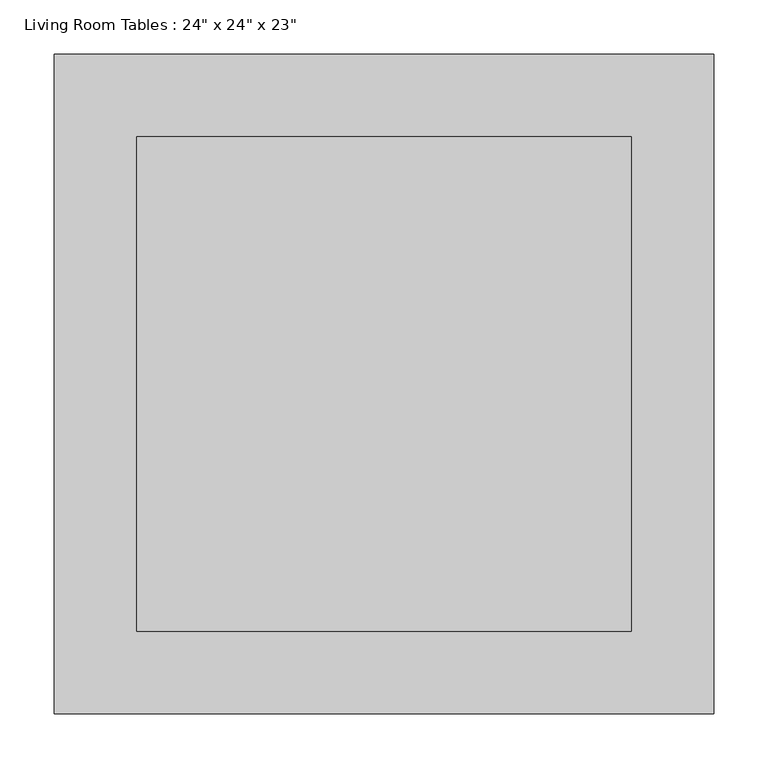
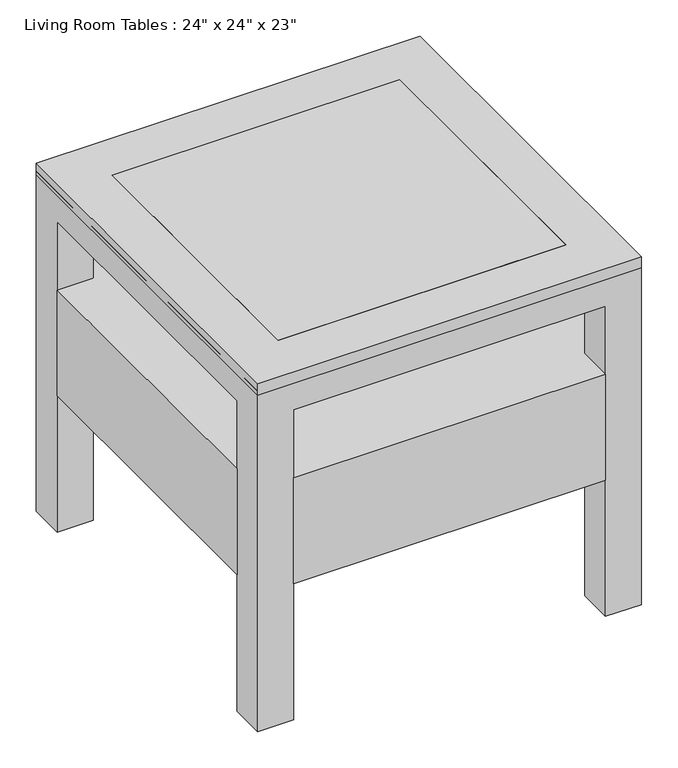
"""IFC4 building model written with IfcOpenShell, lengths in millimetres: furniture geometry."""

from ifc_helpers import new_model, si_unit, frame, origin, place, context, project, spatial, polyline, outline, extrude, faceted_brep, source, transform, mapped, element, save


def furniture_79813b58(model_context):
    return source(origin(), model_context, "Body", "SolidModel", [
        extrude(outline(polyline([(265.9157667, 400.0110778), (265.9157667, 342.8610778), (323.0657667, 342.8610778), (323.0657667, -152.4389222), (265.9157667, -152.4389222), (265.9157667, -209.5889222), (-229.3842333, -209.5889222), (-229.3842333, -152.4389222), (-286.5342333, -152.4389222), (-286.5342333, 342.8610778), (-229.3842333, 342.8610778), (-229.3842333, 400.0110778), (265.9157667, 400.0110778)])), frame((0.0, 0.0, 228.6), z_axis=(0.0, 0.0, 1.0), x_axis=(1.0, 0.0, 0.0)), (0.0, 0.0, 1.0), 177.8),
        extrude(outline(polyline([(246.8657667, 323.8110778), (246.8657667, -133.3889222), (-210.3342333, -133.3889222), (-210.3342333, 323.8110778), (246.8657667, 323.8110778)])), frame((0.0, 0.0, 571.5), z_axis=(0.0, 0.0, 1.0), x_axis=(1.0, 0.0, 0.0)), (0.0, 0.0, 1.0), 12.7),
        extrude(outline(polyline([(323.0657667, 400.0110778), (323.0657667, -209.5889222), (-286.5342333, -209.5889222), (-286.5342333, 400.0110778), (323.0657667, 400.0110778)]), holes=[polyline([(246.8657667, 323.8110778), (-210.3342333, 323.8110778), (-210.3342333, -133.3889222), (246.8657667, -133.3889222), (246.8657667, 323.8110778)])]), frame((0.0, 0.0, 565.15), z_axis=(0.0, 0.0, 1.0), x_axis=(1.0, 0.0, 0.0)), (0.0, 0.0, 1.0), 19.05),
        faceted_brep([(-286.5342333, 400.0110778, 571.5), (-286.5342333, -209.5889222, 571.5), (323.0657667, -209.5889222, 571.5), (323.0657667, 400.0110778, 571.5), (-273.8342333, 342.8610778, 571.5), (-229.3842333, 342.8610778, 571.5), (-229.3842333, 387.3110778, 571.5), (265.9157667, 387.3110778, 571.5), (265.9157667, 342.8610778, 571.5), (310.3657667, 342.8610778, 571.5), (310.3657667, -152.4389222, 571.5), (265.9157667, -152.4389222, 571.5), (265.9157667, -196.8889222, 571.5), (-229.3842333, -196.8889222, 571.5), (-229.3842333, -152.4389222, 571.5), (-273.8342333, -152.4389222, 571.5), (-286.5342333, -152.4389222, 520.7), (-286.5342333, 342.8610778, 520.7), (-273.8342333, 342.8610778, 520.7), (-273.8342333, -152.4389222, 520.7), (-229.3842333, -209.5889222, 520.7), (-229.3842333, -196.8889222, 520.7), (265.9157667, -196.8889222, 520.7), (265.9157667, -209.5889222, 520.7), (-229.3842333, 387.3110778, 520.7), (-229.3842333, 400.0110778, 520.7), (265.9157667, 400.0110778, 520.7), (265.9157667, 387.3110778, 520.7), (323.0657667, 342.8610778, 520.7), (323.0657667, -152.4389222, 520.7), (310.3657667, -152.4389222, 520.7), (310.3657667, 342.8610778, 520.7), (323.0657667, 400.0110778, 0.0), (265.9157667, 400.0110778, 0.0), (-229.3842333, 400.0110778, 0.0), (-286.5342333, 400.0110778, 0.0), (-286.5342333, 342.8610778, 0.0), (-286.5342333, -152.4389222, 0.0), (-286.5342333, -209.5889222, 0.0), (-229.3842333, -209.5889222, 0.0), (265.9157667, -209.5889222, 0.0), (323.0657667, -209.5889222, 0.0), (323.0657667, -152.4389222, 0.0), (323.0657667, 342.8610778, 0.0), (-229.3842333, 342.8610778, 0.0), (-229.3842333, -152.4389222, 0.0), (265.9157667, 342.8610778, 0.0), (265.9157667, -152.4389222, 0.0)], [[[0, 1, 2, 3], [4, 5, 6, 7, 8, 9, 10, 11, 12, 13, 14, 15]], [[16, 17, 18, 19]], [[20, 21, 22, 23]], [[24, 25, 26, 27]], [[28, 29, 30, 31]], [[0, 3, 32, 33, 26, 25, 34, 35]], [[35, 36, 17, 16, 37, 38, 1, 0]], [[2, 1, 38, 39, 20, 23, 40, 41]], [[32, 3, 2, 41, 42, 29, 28, 43]], [[4, 15, 19, 18]], [[6, 24, 27, 7]], [[10, 9, 31, 30]], [[21, 13, 12, 22]], [[5, 44, 34, 25, 24, 6]], [[39, 45, 14, 13, 21, 20]], [[36, 35, 34, 44]], [[44, 5, 4, 18, 17, 36]], [[14, 45, 37, 16, 19, 15]], [[38, 37, 45, 39]], [[33, 46, 8, 7, 27, 26]], [[11, 47, 40, 23, 22, 12]], [[46, 33, 32, 43]], [[8, 46, 43, 28, 31, 9]], [[47, 11, 10, 30, 29, 42]], [[40, 47, 42, 41]]]),
    ])


if __name__ == "__main__":
    model = new_model("IFC4")
    model_context = context("Model", 3, world=origin())
    ifc_project = project(units=[si_unit("LENGTHUNIT", "METRE", prefix="MILLI")], contexts=[model_context])
    site = spatial("IfcSite", under=ifc_project)
    building = spatial("IfcBuilding", under=site)
    placement = place(None, origin())
    furniture_shape = furniture_79813b58(model_context)
    element("IfcFurniture", 1, ObjectType="Living Room Tables : 24\" x 24\" x 23\"", at=placement, inside=building, context=model_context, shape_type="MappedRepresentation", body=[
        mapped(furniture_shape, transform((0.0, 0.0, 0.0), x_axis=(1.0, 0.0, 0.0), y_axis=(0.0, 1.0, 0.0), z_axis=(0.0, 0.0, 1.0))),
    ])
    save(model, "model.ifc")

# Revit data of these elements
# Type "Living Room Tables : 24\" x 24\" x 23\""
#   Assembly Code = "E2020200"
#   Post Width = 0' - 2 1/4"
#   Framing Thickness = 0' - 0 1/2"
#   Drawer Top Height = 1' - 0"
#   Border Thickness = 0' - 3"
#   Height = 1' - 11"
#   Length = 2' - 0"
#   Width = 2' - 0"
#   Top Material = Metal - Chrome
#   Frame Material = Wood - Teak
# Element 1 (IfcFurniture, "Living Room Tables : 24\" x 24\" x 23\"")
#   Materials on its faces: "Wood - Teak", "Glass - Clear, Grey"
# Materials
#   "Metal - Chrome": class "Metal", colour RGB 244 244 244, transparency 0, Comments = "Rendering appearance not upgraded Rendering appearance not upgraded ", Description = "Chrome"
#   "Wood - Teak": class "Wood", colour RGB 145 112 90, transparency 0
#   "Glass - Clear, Grey": class "Glass", colour RGB 252 255 255, transparency 0.64, Comments = "Rendering appearance not upgraded Rendering appearance not upgraded "
